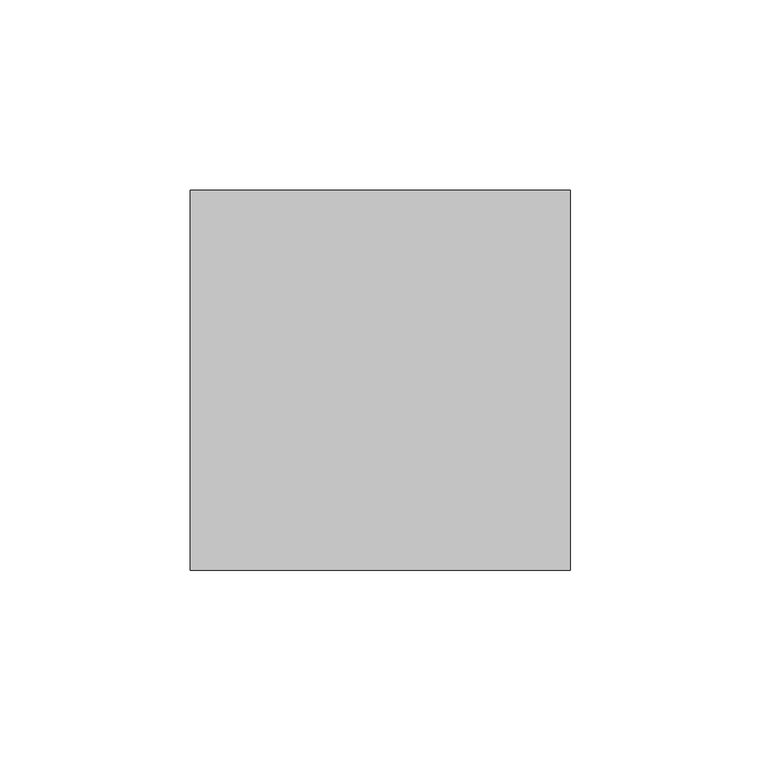
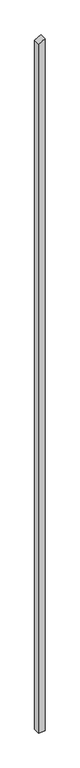
"""IFC4 building model written with IfcOpenShell, lengths in millimetres: column geometry, Holzstütze 159706 : Holzstütze 159706."""

from ifc_helpers import new_model, si_unit, frame, origin, place, context, project, spatial, polyline, outline, extrude, source, transform, mapped, element, save


def column_0947067b(model_context):
    return source(origin(), model_context, "Body", "SweptSolid", [
        extrude(outline(polyline([(-500.0, 165627.7593015), (-500.0, 165727.7593015), (10641.011365, 165727.7593015), (10590.0588201, 165627.7593015), (-500.0, 165627.7593015)])), frame((0.0, 26981.9343946, 0.0), z_axis=(0.0, 1.0, 0.0), x_axis=(0.0, 0.0, 1.0)), (0.0, 0.0, 1.0), 100.0),
    ])


if __name__ == "__main__":
    model = new_model("IFC4")
    model_context = context("Model", 3, world=origin())
    ifc_project = project(units=[si_unit("LENGTHUNIT", "METRE", prefix="MILLI")], contexts=[model_context])
    site = spatial("IfcSite", under=ifc_project)
    building = spatial("IfcBuilding", under=site)
    placement = place(None, origin())
    column_shape = column_0947067b(model_context)
    element("IfcColumn", 1, ObjectType="Holzstütze 159706 : Holzstütze 159706", at=placement, inside=building, context=model_context, shape_type="MappedRepresentation", body=[
        mapped(column_shape, transform((0.0, 0.0, 0.0), x_axis=(1.0, 0.0, 0.0), y_axis=(0.0, 1.0, 0.0), z_axis=(0.0, 0.0, 1.0))),
    ])
    save(model, "model.ifc")

# Revit data of these elements
# Type "Holzstütze 159706 : Holzstütze 159706"
#   Abrechnungsart = "m"
#   Allright_Bauteil_ID = "0152St 0000143522"
#   Bezeichnung = "Holzstütze"
#   Codetext = "ST-HOLZ\\"
#   Gewerk = "Zimmer- und Holzbauarbeiten"
#   Material = "Holz"
#   Objektname = "Stütze"
#   NameOverride = "Holzstütze"
#   Reference = "Holzstütze"
#   Status = "NEW"
#   ThermalTransmittance = 0.0000 BTU/(h·ft²·°F)
#   Roll = 0.00°
#   Slope = 0.00°
#   2D Interaktion = yes
#   IsExternal = yes
#   LoadBearing = yes
# Element 1 (IfcColumn, "Holzstütze 159706 : Holzstütze 159706")
#   Materials on its faces: "holzschalung"
# Materials
#   "holzschalung": class "Unassigned", colour RGB 128 128 128, transparency 0
